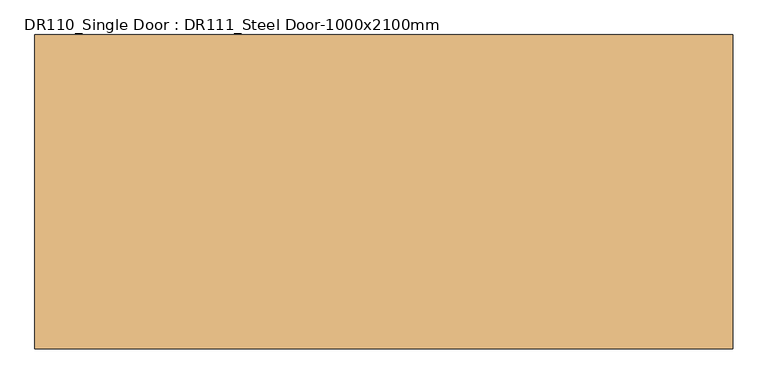
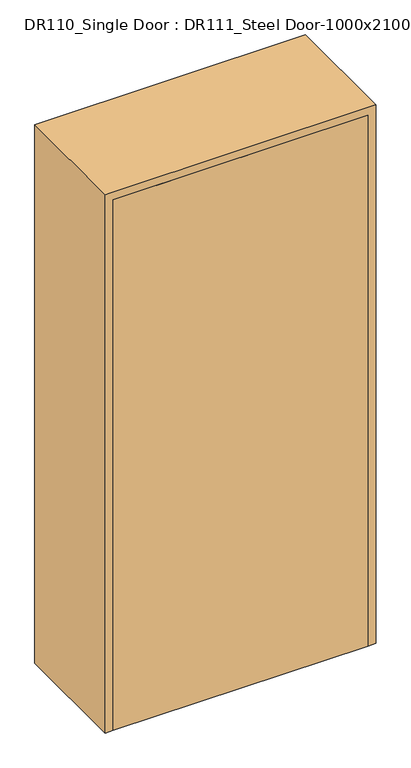
"""IFC4 building model written with IfcOpenShell, lengths in millimetres: door geometry, DR110_Single Door : DR111_Steel Door-1000x2100mm."""

import ifcopenshell
import ifcopenshell.guid

model = None  # the IFC model being written
_history = None  # IfcOwnerHistory: only IFC2X3 demands one
_inside = {}  # id of a spatial element -> (the spatial element, [elements in it])
_under = {}  # id of a project, library or spatial element -> (it, [spatial elements below it])
_declared = {}  # id of a project -> (the project, [libraries it declares])
_typed = {}  # id of a type object -> (the type object, [elements of that type])
_made_of = {}  # id of a material, layer set ... -> (it, [elements and type objects made of it])


def new_model(schema):
    """Start an empty IFC model of exactly this schema.

    Asked for "IFC4X3", IfcOpenShell would pick the latest addendum, in which some entities
    have other attributes; the version numbers below select the first issue.
    IFC2X3 requires an IfcOwnerHistory on every rooted entity: one is made here for all.
    """
    global model, _history
    if schema == "IFC4X3":
        model = ifcopenshell.file(schema_version=(4, 3, 0, 0))
    else:
        model = ifcopenshell.file(schema=schema)
    _inside.clear()
    _under.clear()
    _declared.clear()
    _typed.clear()
    _made_of.clear()
    _history = None
    if model.schema == "IFC2X3":
        org = make("IfcOrganization", Name="unknown")
        user = make(
            "IfcPersonAndOrganization",
            ThePerson=make("IfcPerson", FamilyName="unknown"),
            TheOrganization=org,
        )
        app = make(
            "IfcApplication",
            ApplicationDeveloper=org,
            Version="unknown",
            ApplicationFullName="unknown",
            ApplicationIdentifier="unknown",
        )
        _history = make(
            "IfcOwnerHistory",
            OwningUser=user,
            OwningApplication=app,
            ChangeAction="ADDED",
            CreationDate=0,
        )
    return model


def make(cls, **values):
    """One entity of the class cls with the attributes given. An attribute that is None is left unset."""
    return model.create_entity(
        cls, **{name: value for name, value in values.items() if value is not None}
    )


def rooted(cls, **values):
    """An entity with a GlobalId (a new one), such as an element, a storey or a relation."""
    return make(cls, GlobalId=ifcopenshell.guid.new(), OwnerHistory=_history, **values)


def si_unit(unit_type, name, prefix=None):
    """IfcSIUnit, for example si_unit("LENGTHUNIT", "METRE", prefix="MILLI")."""
    return make("IfcSIUnit", UnitType=unit_type, Prefix=prefix, Name=name)


def assignment(units):
    """IfcUnitAssignment: the units of a project."""
    return None if units is None else make("IfcUnitAssignment", Units=units)


def point(xyz):
    """IfcCartesianPoint."""
    return None if xyz is None else make("IfcCartesianPoint", Coordinates=xyz)


def direction(xyz):
    """IfcDirection."""
    return None if xyz is None else make("IfcDirection", DirectionRatios=xyz)


def frame(location, z_axis=None, x_axis=None):
    """IfcAxis2Placement3D, a coordinate frame: its origin and axes. An axis left out is left unset."""
    return make(
        "IfcAxis2Placement3D",
        Location=point(location),
        Axis=direction(z_axis),
        RefDirection=direction(x_axis),
    )


def origin():
    """The frame at (0, 0, 0) with its axes left unset."""
    return frame((0.0, 0.0, 0.0))


def origin_with_axes():
    """The frame at (0, 0, 0) with the z axis (0, 0, 1) and the x axis (1, 0, 0) written out."""
    return frame((0.0, 0.0, 0.0), z_axis=(0.0, 0.0, 1.0), x_axis=(1.0, 0.0, 0.0))


def place(relative_to, where):
    """IfcLocalPlacement: puts the frame where relative to a parent placement (None: the world)."""
    return make(
        "IfcLocalPlacement", PlacementRelTo=relative_to, RelativePlacement=where
    )


def context(
    kind, dimensions, precision=None, world=None, true_north=None, identifier=None
):
    """IfcGeometricRepresentationContext, for example the 3D "Model" context."""
    return make(
        "IfcGeometricRepresentationContext",
        ContextIdentifier=identifier,
        ContextType=kind,
        CoordinateSpaceDimension=dimensions,
        Precision=precision,
        WorldCoordinateSystem=world,
        TrueNorth=true_north,
    )


def project(units=None, contexts=None):
    """IfcProject with its units and contexts."""
    return rooted(
        "IfcProject",
        Name="project",
        RepresentationContexts=contexts,
        UnitsInContext=assignment(units),
    )


def spatial(cls, under=None, at=None, **own):
    """A site, building, storey or space (cls), placed at a placement, below another one or the project."""
    s = rooted(cls, ObjectPlacement=at, **own)
    if under is not None:
        _under.setdefault(under.id(), (under, []))[1].append(s)
    return s


def polyline(points):
    """IfcPolyline through the points."""
    return make("IfcPolyline", Points=[point(p) for p in points])


def outline(outer, holes=None, kind="AREA"):
    """IfcArbitraryClosedProfileDef: a profile drawn as a closed curve; with holes, ...WithVoids."""
    if holes is None:
        return make("IfcArbitraryClosedProfileDef", ProfileType=kind, OuterCurve=outer)
    return make(
        "IfcArbitraryProfileDefWithVoids",
        ProfileType=kind,
        OuterCurve=outer,
        InnerCurves=holes,
    )


def extrude(swept, where, along, depth):
    """IfcExtrudedAreaSolid: the profile swept, set in the frame where, extruded along a direction by depth."""
    return make(
        "IfcExtrudedAreaSolid",
        SweptArea=swept,
        Position=where,
        ExtrudedDirection=direction(along),
        Depth=depth,
    )


def faces_of(points, faces, orient=None, outer=None):
    """IfcFace entities. A face is a list of loops; a loop is a list of indices into points, from 0.

    orient and outer hold one flag for each loop. By default every Orientation is true, the
    first loop of a face is its IfcFaceOuterBound and the others are IfcFaceBound.
    """
    made = []
    for i, loops in enumerate(faces):
        bounds = []
        for j, loop in enumerate(loops):
            is_outer = j == 0 if outer is None else outer[i][j]
            bounds.append(
                make(
                    "IfcFaceOuterBound" if is_outer else "IfcFaceBound",
                    Bound=make("IfcPolyLoop", Polygon=[points[k] for k in loop]),
                    Orientation=True if orient is None else orient[i][j],
                )
            )
        made.append(make("IfcFace", Bounds=bounds))
    return made


def faceted_brep(points, faces, orient=None, outer=None, voids=None):
    """IfcFacetedBrep: a solid bounded by flat faces; with voids (closed shells), ...WithVoids."""
    shared = [point(p) for p in points]
    hull = make("IfcClosedShell", CfsFaces=faces_of(shared, faces, orient, outer))
    if voids is None:
        return make("IfcFacetedBrep", Outer=hull)
    return make(
        "IfcFacetedBrepWithVoids",
        Outer=hull,
        Voids=[
            make(cls, CfsFaces=faces_of(shared, fs, o, b)) for cls, fs, o, b in voids
        ],
    )


def shape(context_of_items, identifier, shape_type, items):
    """IfcShapeRepresentation: the items that make up one representation, for example the "Body"."""
    return make(
        "IfcShapeRepresentation",
        ContextOfItems=context_of_items,
        RepresentationIdentifier=identifier,
        RepresentationType=shape_type,
        Items=items,
    )


def source(mapping_origin, context_of_items, identifier, shape_type, items):
    """IfcRepresentationMap: a shape defined once, which mapped items show again and again."""
    return make(
        "IfcRepresentationMap",
        MappingOrigin=mapping_origin,
        MappedRepresentation=shape(context_of_items, identifier, shape_type, items),
    )


def transform(
    local_origin,
    x_axis=None,
    y_axis=None,
    z_axis=None,
    scale=None,
    scale2=None,
    scale3=None,
    uniform=True,
):
    """IfcCartesianTransformationOperator3D, or its non-uniform kind. x_axis, y_axis, z_axis: its Axis1, 2, 3."""
    if uniform:
        return make(
            "IfcCartesianTransformationOperator3D",
            Axis1=direction(x_axis),
            Axis2=direction(y_axis),
            LocalOrigin=point(local_origin),
            Scale=scale,
            Axis3=direction(z_axis),
        )
    return make(
        "IfcCartesianTransformationOperator3DnonUniform",
        Axis1=direction(x_axis),
        Axis2=direction(y_axis),
        LocalOrigin=point(local_origin),
        Scale=scale,
        Axis3=direction(z_axis),
        Scale2=scale2,
        Scale3=scale3,
    )


def mapped(mapping_source, mapping_target):
    """IfcMappedItem: shows the shape of a source again, moved by a transform."""
    return make(
        "IfcMappedItem", MappingSource=mapping_source, MappingTarget=mapping_target
    )


def made_of(thing, what):
    """Note that an element or type object is made of a material, layer set ...; save() writes the relation."""
    if what is not None:
        _made_of.setdefault(what.id(), (what, []))[1].append(thing)
    return thing


def element(
    cls,
    number,
    at=None,
    inside=None,
    cuts=None,
    type_object=None,
    material=None,
    context=None,
    identifier="Body",
    shape_type=None,
    held_by="IfcProductDefinitionShape",
    body=None,
    shapes=None,
    **own,
):
    """One element of the class cls, such as IfcWall. Its Tag is "e" and its number.

    at: its placement. inside: the storey or other place that contains it. cuts: it is an
    opening in that element (IfcRelVoidsElement). A single representation is given by context,
    identifier, shape_type and body (its items); several are given by shapes. held_by: the class
    of the entity that holds the representations. save() writes the other relations.
    """
    e = rooted(cls, Tag="e%d" % number, ObjectPlacement=at, **own)
    if body is not None:
        shapes = [shape(context, identifier, shape_type, body)]
    if shapes is not None:
        e.Representation = make(held_by, Representations=shapes)
    if inside is not None:
        _inside.setdefault(inside.id(), (inside, []))[1].append(e)
    if cuts is not None:
        rooted(
            "IfcRelVoidsElement", RelatingBuildingElement=cuts, RelatedOpeningElement=e
        )
    if type_object is not None:
        _typed.setdefault(type_object.id(), (type_object, []))[1].append(e)
    return made_of(e, material)


def aggregate(whole, parts):
    """IfcRelAggregates: a whole, such as a stair, and the parts it consists of."""
    return rooted("IfcRelAggregates", RelatingObject=whole, RelatedObjects=parts)


def save(model, path):
    """Write the relations noted so far, then the file.

    IfcRelAggregates (storeys below a building ...), IfcRelContainedInSpatialStructure (elements
    in a storey), IfcRelDefinesByType, IfcRelAssociatesMaterial and IfcRelDeclares: one each for
    every whole, place, type object, material and project.
    """
    for whole, parts in _under.values():
        aggregate(whole, parts)
    for where, things in _inside.values():
        rooted(
            "IfcRelContainedInSpatialStructure",
            RelatedElements=things,
            RelatingStructure=where,
        )
    for kind, things in _typed.values():
        rooted("IfcRelDefinesByType", RelatedObjects=things, RelatingType=kind)
    for what, things in _made_of.values():
        rooted("IfcRelAssociatesMaterial", RelatedObjects=things, RelatingMaterial=what)
    for by, libraries in _declared.values():
        rooted("IfcRelDeclares", RelatingContext=by, RelatedDefinitions=libraries)
    model.write(path)


def dr110_single_door_dr111_steel_door_1000x2100mm_3adf1b50(model_context):
    return source(origin(), model_context, "Body", "SolidModel", [
        extrude(outline(polyline([(470.0, -225.0), (-470.0, -225.0), (-470.0, -190.0), (470.0, -190.0), (470.0, -225.0)])), origin_with_axes(), (0.0, 0.0, 1.0), 2070.0),
        faceted_brep([(470.0, -225.0, 0.0), (470.0, -190.0, 0.0), (450.0, -190.0, 0.0), (450.0, 190.0, 0.0), (470.0, 190.0, 0.0), (470.0, 225.0, 0.0), (500.0, 225.0, 0.0), (500.0, -225.0, 0.0), (500.0, -225.0, 2100.0), (-500.0, -225.0, 2100.0), (-500.0, -225.0, 0.0), (-470.0, -225.0, 0.0), (-470.0, -225.0, 2070.0), (470.0, -225.0, 2070.0), (500.0, 225.0, 2100.0), (470.0, 225.0, 2070.0), (-470.0, 225.0, 2070.0), (-470.0, 225.0, 0.0), (-500.0, 225.0, 0.0), (-500.0, 225.0, 2100.0), (470.0, 190.0, 2070.0), (450.0, 190.0, 2050.0), (-450.0, 190.0, 2050.0), (-450.0, 190.0, 0.0), (-470.0, 190.0, 0.0), (-470.0, 190.0, 2070.0), (450.0, -190.0, 2050.0), (470.0, -190.0, 2070.0), (-470.0, -190.0, 2070.0), (-470.0, -190.0, 0.0), (-450.0, -190.0, 0.0), (-450.0, -190.0, 2050.0)], [[[0, 1, 2, 3, 4, 5, 6, 7]], [[7, 8, 9, 10, 11, 12, 13, 0]], [[6, 14, 8, 7]], [[5, 15, 16, 17, 18, 19, 14, 6]], [[4, 20, 15, 5]], [[3, 21, 22, 23, 24, 25, 20, 4]], [[2, 26, 21, 3]], [[1, 27, 28, 29, 30, 31, 26, 2]], [[0, 13, 27, 1]], [[12, 11, 29, 28]], [[11, 10, 18, 17, 24, 23, 30, 29]], [[19, 18, 10, 9]], [[25, 24, 17, 16]], [[31, 30, 23, 22]], [[14, 19, 9, 8]], [[20, 25, 16, 15]], [[26, 31, 22, 21]], [[13, 12, 28, 27]]]),
    ])


if __name__ == "__main__":
    model = new_model("IFC4")
    model_context = context("Model", 3, world=origin())
    ifc_project = project(units=[si_unit("LENGTHUNIT", "METRE", prefix="MILLI")], contexts=[model_context])
    site = spatial("IfcSite", under=ifc_project)
    building = spatial("IfcBuilding", under=site)
    placement = place(None, origin())
    dr110_single_door_dr111_steel_door_1000x2100mm_shape = dr110_single_door_dr111_steel_door_1000x2100mm_3adf1b50(model_context)
    element("IfcDoor", 1, ObjectType="DR110_Single Door : DR111_Steel Door-1000x2100mm", at=placement, inside=building, context=model_context, shape_type="MappedRepresentation", body=[
        mapped(dr110_single_door_dr111_steel_door_1000x2100mm_shape, transform((0.0, 0.0, 0.0), x_axis=(1.0, 0.0, 0.0), y_axis=(0.0, 1.0, 0.0), z_axis=(0.0, 0.0, 1.0))),
    ])
    save(model, "model.ifc")

# Revit data of these elements
# Project information
#   Building Name = "MAIN GATE SECURITY BUILDING"
#   Project Status = "Project Status"
#   Client Name = "현대엔지니어링"
#   Project Address = "서울시 종로구 율곡로 75(계동)"
#   Project Name = "Therma Visayas Energy Project"
#   Project Number = "-"
# Type "DR110_Single Door : DR111_Steel Door-1000x2100mm"
#   Type Mark = "SD"
#   Analytic Construction = "<None>"
#   프레임 투영 외부. = 25 mm
#   프레임 투영 내부. = 25 mm
#   프레임 폭 = 75 mm
#   Height = 2100 mm
#   Width = 1000 mm
#   Define Thermal Properties by = 1
#   문 패널 = SD1 문 패널
#   문 프레임 = A04AQ098-00002_Steel Door_non FP_single
#   Function = (empty or 0)
#   Wall Closure = (empty or 0)
# Element 1 (IfcDoor, "DR110_Single Door : DR111_Steel Door-1000x2100mm")
#   Materials on its faces: "A04AQ098-00002_Steel Door_non FP_single", "SD1 문 패널"
# Materials
#   "SD1 문 패널": class "금속", colour RGB 247 247 247, transparency 0, Description = "STEEL DOOR (1000Wx2100H)"
#   "A04AQ098-00002_Steel Door_non FP_single": class "금속", colour RGB 247 247 247, transparency 0, Description = "Steel Door", W00) Work Master Code = "A04AQ098-00002", W01) Work Master_Lv1 = "Finishing Work", W02) Work Master_Lv2 = "Door & Window Work", W03) Work Master_Spec.1 = "Steel Door w/ Steel Frame", W04) Work Master_Spec.2 = "Fire Protective Rating: N/A, Single Door", W05) Work Master_Spec.3 = "w/ Hardware & Accessories", Cost = 0
